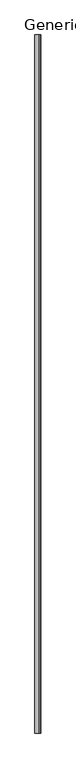
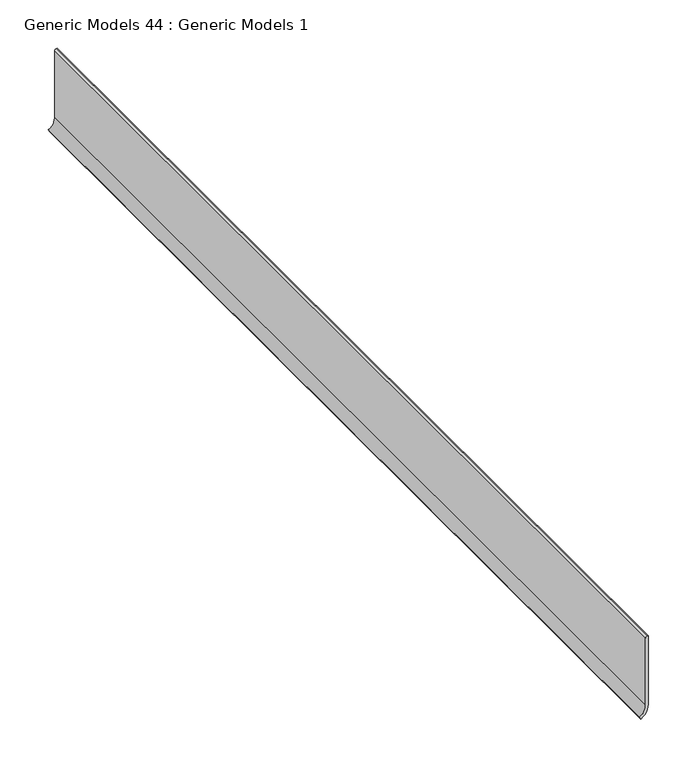
"""IFC4 building model written with IfcOpenShell, lengths in millimetres: proxy geometry, Generic Models 44 : Generic Models 1."""

import ifcopenshell
import ifcopenshell.guid

model = None  # the IFC model being written
_history = None  # IfcOwnerHistory: only IFC2X3 demands one
_inside = {}  # id of a spatial element -> (the spatial element, [elements in it])
_under = {}  # id of a project, library or spatial element -> (it, [spatial elements below it])
_declared = {}  # id of a project -> (the project, [libraries it declares])
_typed = {}  # id of a type object -> (the type object, [elements of that type])
_made_of = {}  # id of a material, layer set ... -> (it, [elements and type objects made of it])


def new_model(schema):
    """Start an empty IFC model of exactly this schema.

    Asked for "IFC4X3", IfcOpenShell would pick the latest addendum, in which some entities
    have other attributes; the version numbers below select the first issue.
    IFC2X3 requires an IfcOwnerHistory on every rooted entity: one is made here for all.
    """
    global model, _history
    if schema == "IFC4X3":
        model = ifcopenshell.file(schema_version=(4, 3, 0, 0))
    else:
        model = ifcopenshell.file(schema=schema)
    _inside.clear()
    _under.clear()
    _declared.clear()
    _typed.clear()
    _made_of.clear()
    _history = None
    if model.schema == "IFC2X3":
        org = make("IfcOrganization", Name="unknown")
        user = make(
            "IfcPersonAndOrganization",
            ThePerson=make("IfcPerson", FamilyName="unknown"),
            TheOrganization=org,
        )
        app = make(
            "IfcApplication",
            ApplicationDeveloper=org,
            Version="unknown",
            ApplicationFullName="unknown",
            ApplicationIdentifier="unknown",
        )
        _history = make(
            "IfcOwnerHistory",
            OwningUser=user,
            OwningApplication=app,
            ChangeAction="ADDED",
            CreationDate=0,
        )
    return model


def make(cls, **values):
    """One entity of the class cls with the attributes given. An attribute that is None is left unset."""
    return model.create_entity(
        cls, **{name: value for name, value in values.items() if value is not None}
    )


def rooted(cls, **values):
    """An entity with a GlobalId (a new one), such as an element, a storey or a relation."""
    return make(cls, GlobalId=ifcopenshell.guid.new(), OwnerHistory=_history, **values)


def si_unit(unit_type, name, prefix=None):
    """IfcSIUnit, for example si_unit("LENGTHUNIT", "METRE", prefix="MILLI")."""
    return make("IfcSIUnit", UnitType=unit_type, Prefix=prefix, Name=name)


def assignment(units):
    """IfcUnitAssignment: the units of a project."""
    return None if units is None else make("IfcUnitAssignment", Units=units)


def point(xyz):
    """IfcCartesianPoint."""
    return None if xyz is None else make("IfcCartesianPoint", Coordinates=xyz)


def direction(xyz):
    """IfcDirection."""
    return None if xyz is None else make("IfcDirection", DirectionRatios=xyz)


def frame(location, z_axis=None, x_axis=None):
    """IfcAxis2Placement3D, a coordinate frame: its origin and axes. An axis left out is left unset."""
    return make(
        "IfcAxis2Placement3D",
        Location=point(location),
        Axis=direction(z_axis),
        RefDirection=direction(x_axis),
    )


def frame_2d(location, x_axis=None):
    """IfcAxis2Placement2D, a coordinate frame in the plane: its origin and x axis."""
    return make(
        "IfcAxis2Placement2D", Location=point(location), RefDirection=direction(x_axis)
    )


def origin():
    """The frame at (0, 0, 0) with its axes left unset."""
    return frame((0.0, 0.0, 0.0))


def place(relative_to, where):
    """IfcLocalPlacement: puts the frame where relative to a parent placement (None: the world)."""
    return make(
        "IfcLocalPlacement", PlacementRelTo=relative_to, RelativePlacement=where
    )


def context(
    kind, dimensions, precision=None, world=None, true_north=None, identifier=None
):
    """IfcGeometricRepresentationContext, for example the 3D "Model" context."""
    return make(
        "IfcGeometricRepresentationContext",
        ContextIdentifier=identifier,
        ContextType=kind,
        CoordinateSpaceDimension=dimensions,
        Precision=precision,
        WorldCoordinateSystem=world,
        TrueNorth=true_north,
    )


def project(units=None, contexts=None):
    """IfcProject with its units and contexts."""
    return rooted(
        "IfcProject",
        Name="project",
        RepresentationContexts=contexts,
        UnitsInContext=assignment(units),
    )


def spatial(cls, under=None, at=None, **own):
    """A site, building, storey or space (cls), placed at a placement, below another one or the project."""
    s = rooted(cls, ObjectPlacement=at, **own)
    if under is not None:
        _under.setdefault(under.id(), (under, []))[1].append(s)
    return s


def polyline(points):
    """IfcPolyline through the points."""
    return make("IfcPolyline", Points=[point(p) for p in points])


def circle_curve(where, radius):
    """IfcCircle in the frame where."""
    return make("IfcCircle", Position=where, Radius=radius)


def trimmed(basis, trim1, trim2, sense, master):
    """IfcTrimmedCurve: the piece of a basis curve between two trims."""
    return make(
        "IfcTrimmedCurve",
        BasisCurve=basis,
        Trim1=trim1,
        Trim2=trim2,
        SenseAgreement=sense,
        MasterRepresentation=master,
    )


def segment(curve, same_sense, transition):
    """IfcCompositeCurveSegment."""
    return make(
        "IfcCompositeCurveSegment",
        Transition=transition,
        SameSense=same_sense,
        ParentCurve=curve,
    )


def composite_curve(segments, self_intersect=None):
    """IfcCompositeCurve: segments joined end to end."""
    return make("IfcCompositeCurve", Segments=segments, SelfIntersect=self_intersect)


def outline(outer, holes=None, kind="AREA"):
    """IfcArbitraryClosedProfileDef: a profile drawn as a closed curve; with holes, ...WithVoids."""
    if holes is None:
        return make("IfcArbitraryClosedProfileDef", ProfileType=kind, OuterCurve=outer)
    return make(
        "IfcArbitraryProfileDefWithVoids",
        ProfileType=kind,
        OuterCurve=outer,
        InnerCurves=holes,
    )


def extrude(swept, where, along, depth):
    """IfcExtrudedAreaSolid: the profile swept, set in the frame where, extruded along a direction by depth."""
    return make(
        "IfcExtrudedAreaSolid",
        SweptArea=swept,
        Position=where,
        ExtrudedDirection=direction(along),
        Depth=depth,
    )


def shape(context_of_items, identifier, shape_type, items):
    """IfcShapeRepresentation: the items that make up one representation, for example the "Body"."""
    return make(
        "IfcShapeRepresentation",
        ContextOfItems=context_of_items,
        RepresentationIdentifier=identifier,
        RepresentationType=shape_type,
        Items=items,
    )


def source(mapping_origin, context_of_items, identifier, shape_type, items):
    """IfcRepresentationMap: a shape defined once, which mapped items show again and again."""
    return make(
        "IfcRepresentationMap",
        MappingOrigin=mapping_origin,
        MappedRepresentation=shape(context_of_items, identifier, shape_type, items),
    )


def transform(
    local_origin,
    x_axis=None,
    y_axis=None,
    z_axis=None,
    scale=None,
    scale2=None,
    scale3=None,
    uniform=True,
):
    """IfcCartesianTransformationOperator3D, or its non-uniform kind. x_axis, y_axis, z_axis: its Axis1, 2, 3."""
    if uniform:
        return make(
            "IfcCartesianTransformationOperator3D",
            Axis1=direction(x_axis),
            Axis2=direction(y_axis),
            LocalOrigin=point(local_origin),
            Scale=scale,
            Axis3=direction(z_axis),
        )
    return make(
        "IfcCartesianTransformationOperator3DnonUniform",
        Axis1=direction(x_axis),
        Axis2=direction(y_axis),
        LocalOrigin=point(local_origin),
        Scale=scale,
        Axis3=direction(z_axis),
        Scale2=scale2,
        Scale3=scale3,
    )


def mapped(mapping_source, mapping_target):
    """IfcMappedItem: shows the shape of a source again, moved by a transform."""
    return make(
        "IfcMappedItem", MappingSource=mapping_source, MappingTarget=mapping_target
    )


def made_of(thing, what):
    """Note that an element or type object is made of a material, layer set ...; save() writes the relation."""
    if what is not None:
        _made_of.setdefault(what.id(), (what, []))[1].append(thing)
    return thing


def element(
    cls,
    number,
    at=None,
    inside=None,
    cuts=None,
    type_object=None,
    material=None,
    context=None,
    identifier="Body",
    shape_type=None,
    held_by="IfcProductDefinitionShape",
    body=None,
    shapes=None,
    **own,
):
    """One element of the class cls, such as IfcWall. Its Tag is "e" and its number.

    at: its placement. inside: the storey or other place that contains it. cuts: it is an
    opening in that element (IfcRelVoidsElement). A single representation is given by context,
    identifier, shape_type and body (its items); several are given by shapes. held_by: the class
    of the entity that holds the representations. save() writes the other relations.
    """
    e = rooted(cls, Tag="e%d" % number, ObjectPlacement=at, **own)
    if body is not None:
        shapes = [shape(context, identifier, shape_type, body)]
    if shapes is not None:
        e.Representation = make(held_by, Representations=shapes)
    if inside is not None:
        _inside.setdefault(inside.id(), (inside, []))[1].append(e)
    if cuts is not None:
        rooted(
            "IfcRelVoidsElement", RelatingBuildingElement=cuts, RelatedOpeningElement=e
        )
    if type_object is not None:
        _typed.setdefault(type_object.id(), (type_object, []))[1].append(e)
    return made_of(e, material)


def aggregate(whole, parts):
    """IfcRelAggregates: a whole, such as a stair, and the parts it consists of."""
    return rooted("IfcRelAggregates", RelatingObject=whole, RelatedObjects=parts)


def save(model, path):
    """Write the relations noted so far, then the file.

    IfcRelAggregates (storeys below a building ...), IfcRelContainedInSpatialStructure (elements
    in a storey), IfcRelDefinesByType, IfcRelAssociatesMaterial and IfcRelDeclares: one each for
    every whole, place, type object, material and project.
    """
    for whole, parts in _under.values():
        aggregate(whole, parts)
    for where, things in _inside.values():
        rooted(
            "IfcRelContainedInSpatialStructure",
            RelatedElements=things,
            RelatingStructure=where,
        )
    for kind, things in _typed.values():
        rooted("IfcRelDefinesByType", RelatedObjects=things, RelatingType=kind)
    for what, things in _made_of.values():
        rooted("IfcRelAssociatesMaterial", RelatedObjects=things, RelatingMaterial=what)
    for by, libraries in _declared.values():
        rooted("IfcRelDeclares", RelatingContext=by, RelatedDefinitions=libraries)
    model.write(path)


def generic_models_44_generic_models_1_f536fb9f(model_context):
    return source(origin(), model_context, "Body", "SweptSolid", [
        extrude(outline(composite_curve([segment(polyline([(73.749588, 50688.3189813), (73.749588, 50687.2307831)]), True, "CONTINUOUS"), segment(trimmed(circle_curve(frame_2d((71.6627862, 50687.2307831)), 2.0868018), [point((73.749588, 50687.2307831))], [point((71.6627862, 50685.1439813))], False, "CARTESIAN"), True, "CONTINUOUS"), segment(polyline([(71.6627862, 50685.1439813), (-12.4007813, 50685.1439813)]), True, "CONTINUOUS"), segment(trimmed(circle_curve(frame_2d((-12.4007813, 50670.4792845)), 14.6646968), [point((-12.4007813, 50685.1439813))], [point((-25.1007813, 50677.8116329))], True, "CARTESIAN"), True, "CONTINUOUS"), segment(polyline([(-25.1007813, 50677.8116329), (-27.850412, 50679.3991329)]), True, "CONTINUOUS"), segment(trimmed(circle_curve(frame_2d((-12.4007813, 50670.4792845)), 17.8396968), [point((-27.850412, 50679.3991329))], [point((-12.4007813, 50688.3189813))], False, "CARTESIAN"), True, "CONTINUOUS"), segment(polyline([(-12.4007813, 50688.3189813), (73.749588, 50688.3189813)]), True, "CONTINUOUS")], self_intersect=False)), frame((0.0, 0.0, 0.0), z_axis=(0.0, 1.0, 0.0), x_axis=(0.0, 0.0, 1.0)), (0.0, 0.0, 1.0), 1219.2),
    ])


if __name__ == "__main__":
    model = new_model("IFC4")
    model_context = context("Model", 3, world=origin())
    ifc_project = project(units=[si_unit("LENGTHUNIT", "METRE", prefix="MILLI")], contexts=[model_context])
    site = spatial("IfcSite", under=ifc_project)
    building = spatial("IfcBuilding", under=site)
    placement = place(None, origin())
    generic_models_44_generic_models_1_shape = generic_models_44_generic_models_1_f536fb9f(model_context)
    element("IfcBuildingElementProxy", 1, Name="Generic Models 44 : Generic Models 1", ObjectType="Generic Models 44 : Generic Models 1", at=placement, inside=building, context=model_context, shape_type="MappedRepresentation", body=[
        mapped(generic_models_44_generic_models_1_shape, transform((0.0, 0.0, 0.0), x_axis=(1.0, 0.0, 0.0), y_axis=(0.0, 1.0, 0.0), z_axis=(0.0, 0.0, 1.0))),
    ])
    save(model, "model.ifc")

# Revit data of these elements
# Element 1 (IfcBuildingElementProxy, "Generic Models 44 : Generic Models 1")
#   Materials on its faces: "BASE AS SCHEDULED"
# Materials
#   "BASE AS SCHEDULED": class "Generic", colour RGB 120 120 120, transparency 0, Cost = 0
